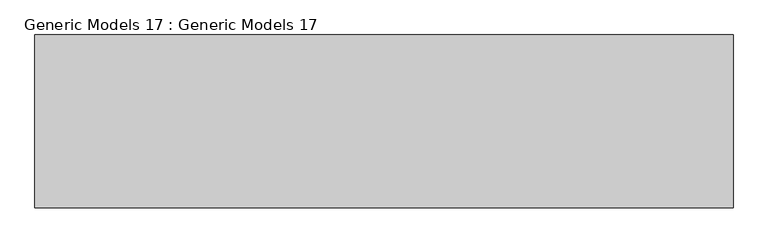
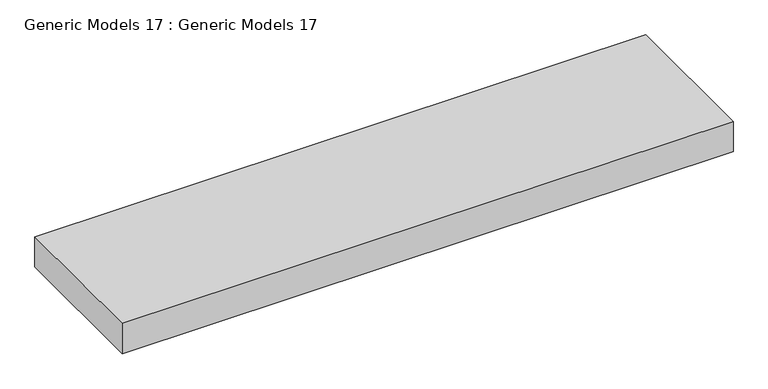
"""IFC4 building model written with IfcOpenShell, lengths in millimetres: proxy geometry, Generic Models 17 : Generic Models 17."""

from ifc_helpers import new_model, si_unit, frame, origin, place, context, project, spatial, polyline, outline, extrude, source, transform, mapped, element, save


def generic_models_17_generic_models_17_8e5ab81f(model_context):
    return source(origin(), model_context, "Body", "SweptSolid", [
        extrude(outline(polyline([(6247.0653137, -5898.1673938), (6247.0653137, -6858.5730338), (2369.8892565, -6858.5730338), (2369.8892565, -5898.1673938), (6247.0653137, -5898.1673938)])), frame((0.0, 0.0, 123551.696), z_axis=(0.0, 0.0, 1.0), x_axis=(1.0, 0.0, 0.0)), (0.0, 0.0, 1.0), 203.2),
    ])


if __name__ == "__main__":
    model = new_model("IFC4")
    model_context = context("Model", 3, world=origin())
    ifc_project = project(units=[si_unit("LENGTHUNIT", "METRE", prefix="MILLI")], contexts=[model_context])
    site = spatial("IfcSite", under=ifc_project)
    building = spatial("IfcBuilding", under=site)
    placement = place(None, origin())
    generic_models_17_generic_models_17_shape = generic_models_17_generic_models_17_8e5ab81f(model_context)
    element("IfcBuildingElementProxy", 1, Name="Generic Models 17 : Generic Models 17", ObjectType="Generic Models 17 : Generic Models 17", at=placement, inside=building, context=model_context, shape_type="MappedRepresentation", body=[
        mapped(generic_models_17_generic_models_17_shape, transform((0.0, 0.0, 0.0), x_axis=(1.0, 0.0, 0.0), y_axis=(0.0, 1.0, 0.0), z_axis=(0.0, 0.0, 1.0))),
    ])
    save(model, "model.ifc")

# Revit data of these elements
# Element 1 (IfcBuildingElementProxy, "Generic Models 17 : Generic Models 17")
#   Materials on its faces: "_CONCRETE SLAB W/ WIRE MESH (SEE STRUCT. DWGS) - POLISHED & SEALED FINISH"
# Materials
#   "_CONCRETE SLAB W/ WIRE MESH (SEE STRUCT. DWGS) - POLISHED & SEALED FINISH": class "Generic", colour RGB 191 191 191, transparency 0, Cost = 0
